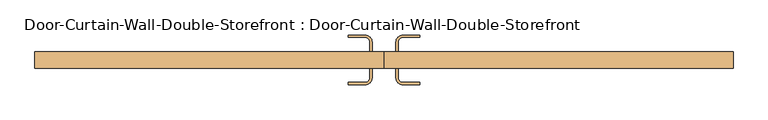
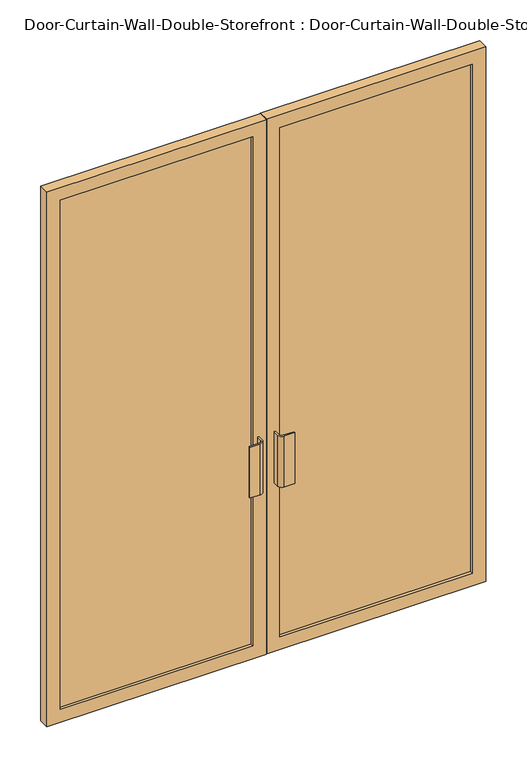
"""IFC4 building model written with IfcOpenShell, lengths in millimetres: door geometry, Door-Curtain-Wall-Double-Storefront : Door-Curtain-Wall-Double-Storefront."""

from ifc_helpers import new_model, si_unit, point, frame, frame_2d, origin, place, context, project, spatial, polyline, circle_curve, trimmed, segment, composite_curve, outline, extrude, source, transform, mapped, element, save


def door_curtain_wall_double_storefront_door_curtain_wall_double_baac0ac5(model_context):
    return source(origin(), model_context, "Body", "SweptSolid", [
        extrude(outline(polyline([(2406.65, 0.7668501), (0.0, 0.7668501), (0.0, 933.45), (2406.65, 933.45), (2406.65, 0.7668501)]), holes=[polyline([(2349.5, 57.9168501), (2349.5, 876.3), (57.15, 876.3), (57.15, 57.9168501), (2349.5, 57.9168501)])]), frame((0.0, -57.15, 0.0), z_axis=(0.0, 1.0, 0.0), x_axis=(0.0, 0.0, 1.0)), (0.0, 0.0, 1.0), 44.45),
        extrude(outline(polyline([(2406.65, -0.8206499), (2406.65, -933.45), (0.0, -933.45), (0.0, -0.8206499), (2406.65, -0.8206499)]), holes=[polyline([(2349.5, -876.3), (2349.5, -57.9706499), (57.15, -57.9706499), (57.15, -876.3), (2349.5, -876.3)])]), frame((0.0, -57.15, 0.0), z_axis=(0.0, 1.0, 0.0), x_axis=(0.0, 0.0, 1.0)), (0.0, 0.0, 1.0), 44.45),
        extrude(outline(polyline([(876.3, -25.4), (876.3, -44.45), (57.9168501, -44.45), (57.9168501, -25.4), (876.3, -25.4)])), frame((0.0, 0.0, 57.15), z_axis=(0.0, 0.0, 1.0), x_axis=(1.0, 0.0, 0.0)), (0.0, 0.0, 1.0), 2292.35),
        extrude(outline(polyline([(-57.9706499, -25.4), (-57.9706499, -44.45), (-876.3, -44.45), (-876.3, -25.4), (-57.9706499, -25.4)])), frame((0.0, 0.0, 57.15), z_axis=(0.0, 0.0, 1.0), x_axis=(1.0, 0.0, 0.0)), (0.0, 0.0, 1.0), 2292.35),
        extrude(outline(composite_curve([segment(polyline([(-31.7768999, 12.7), (-31.7768999, -12.7), (-38.1268999, -12.7), (-38.1268999, 12.7)]), True, "CONTINUOUS"), segment(trimmed(circle_curve(frame_2d((-50.8268999, 12.7)), 12.7), [point((-38.1268999, 12.7))], [point((-50.8268999, 25.4))], True, "CARTESIAN"), True, "CONTINUOUS"), segment(polyline([(-50.8268999, 25.4), (-95.2768999, 25.4), (-95.2768999, 31.75), (-50.8268999, 31.75)]), True, "CONTINUOUS"), segment(trimmed(circle_curve(frame_2d((-50.8268999, 12.7)), 19.05), [point((-50.8268999, 31.75))], [point((-31.7768999, 12.7))], False, "CARTESIAN"), True, "CONTINUOUS")], self_intersect=False)), frame((0.0, 0.0, 762.0), z_axis=(0.0, 0.0, 1.0), x_axis=(1.0, 0.0, 0.0)), (0.0, 0.0, 1.0), 228.6),
        extrude(outline(composite_curve([segment(trimmed(circle_curve(frame_2d((50.7731001, 12.7)), 19.05), [point((31.7231001, 12.7))], [point((50.7731001, 31.75))], False, "CARTESIAN"), True, "CONTINUOUS"), segment(polyline([(50.7731001, 31.75), (95.2231001, 31.75), (95.2231001, 25.4), (50.7731001, 25.4)]), True, "CONTINUOUS"), segment(trimmed(circle_curve(frame_2d((50.7731001, 12.7)), 12.7), [point((50.7731001, 25.4))], [point((38.0731001, 12.7))], True, "CARTESIAN"), True, "CONTINUOUS"), segment(polyline([(38.0731001, 12.7), (38.0731001, -12.7), (31.7231001, -12.7), (31.7231001, 12.7)]), True, "CONTINUOUS")], self_intersect=False)), frame((0.0, 0.0, 762.0), z_axis=(0.0, 0.0, 1.0), x_axis=(1.0, 0.0, 0.0)), (0.0, 0.0, 1.0), 228.6),
        extrude(outline(composite_curve([segment(trimmed(circle_curve(frame_2d((-50.8268999, -82.55)), 19.05), [point((-31.7768999, -82.55))], [point((-50.8268999, -101.6))], False, "CARTESIAN"), True, "CONTINUOUS"), segment(polyline([(-50.8268999, -101.6), (-95.2768999, -101.6), (-95.2768999, -95.25), (-50.8268999, -95.25)]), True, "CONTINUOUS"), segment(trimmed(circle_curve(frame_2d((-50.8268999, -82.55)), 12.7), [point((-50.8268999, -95.25))], [point((-38.1268999, -82.55))], True, "CARTESIAN"), True, "CONTINUOUS"), segment(polyline([(-38.1268999, -82.55), (-38.1268999, -57.15), (-31.7768999, -57.15), (-31.7768999, -82.55)]), True, "CONTINUOUS")], self_intersect=False)), frame((0.0, 0.0, 762.0), z_axis=(0.0, 0.0, 1.0), x_axis=(1.0, 0.0, 0.0)), (0.0, 0.0, 1.0), 228.6),
        extrude(outline(composite_curve([segment(polyline([(31.7231001, -82.55), (31.7231001, -57.15), (38.0731001, -57.15), (38.0731001, -82.55)]), True, "CONTINUOUS"), segment(trimmed(circle_curve(frame_2d((50.7731001, -82.55)), 12.7), [point((38.0731001, -82.55))], [point((50.7731001, -95.25))], True, "CARTESIAN"), True, "CONTINUOUS"), segment(polyline([(50.7731001, -95.25), (95.2231001, -95.25), (95.2231001, -101.6), (50.7731001, -101.6)]), True, "CONTINUOUS"), segment(trimmed(circle_curve(frame_2d((50.7731001, -82.55)), 19.05), [point((50.7731001, -101.6))], [point((31.7231001, -82.55))], False, "CARTESIAN"), True, "CONTINUOUS")], self_intersect=False)), frame((0.0, 0.0, 762.0), z_axis=(0.0, 0.0, 1.0), x_axis=(1.0, 0.0, 0.0)), (0.0, 0.0, 1.0), 228.6),
    ])


if __name__ == "__main__":
    model = new_model("IFC4")
    model_context = context("Model", 3, world=origin())
    ifc_project = project(units=[si_unit("LENGTHUNIT", "METRE", prefix="MILLI")], contexts=[model_context])
    site = spatial("IfcSite", under=ifc_project)
    building = spatial("IfcBuilding", under=site)
    placement = place(None, origin())
    door_curtain_wall_double_storefront_door_curtain_wall_double_shape = door_curtain_wall_double_storefront_door_curtain_wall_double_baac0ac5(model_context)
    element("IfcDoor", 1, ObjectType="Door-Curtain-Wall-Double-Storefront : Door-Curtain-Wall-Double-Storefront", at=placement, inside=building, context=model_context, shape_type="MappedRepresentation", body=[
        mapped(door_curtain_wall_double_storefront_door_curtain_wall_double_shape, transform((0.0, 0.0, 0.0), x_axis=(1.0, 0.0, 0.0), y_axis=(0.0, 1.0, 0.0), z_axis=(0.0, 0.0, 1.0))),
    ])
    save(model, "model.ifc")

# Revit data of these elements
# Type "Door-Curtain-Wall-Double-Storefront : Door-Curtain-Wall-Double-Storefront"
#   Type Mark = "15"
#   Construction Type Id = "opn-d46"
#   Assembly Code = "B2030100"
#   Analytic Construction = "Metal frame, double glass door"
#   Width [instance default] = 6' - 0"
#   Thermal Resistance (R) = 1.3794 (h·ft²·°F)/BTU
#   Swing Angle [instance default] = 90.00°
#   Panel Width [instance default] = 3' - 0"
#   Offset = 0' - 2 1/4"
#   Heat Transfer Coefficient (U) = 0.7250 BTU/(h·ft²·°F)
#   Define Thermal Properties by = 1
#   Function = 1
#   Frame Material = Aluminum
#   Door Handle Material = Aluminum
#   Glazing = Glass
#   Visual Light Transmittance = 0
#   Solar Heat Gain Coefficient = 0
# Element 1 (IfcDoor, "Door-Curtain-Wall-Double-Storefront : Door-Curtain-Wall-Double-Storefront")
#   Width = 6' - 1 1/2"
#   Panel Width = 3' - 0 3/4"
#   Materials on its faces: "Aluminum", "Glass"
# Materials
#   "Aluminum": class "Metal", colour RGB 247 247 247, transparency 0, Description = "Aluminum 6061", Cost = 0
#   "Glass": class "Glass", colour RGB 0 0 255, transparency 0.75, Description = "Soda Lime Glass", Cost = 0
